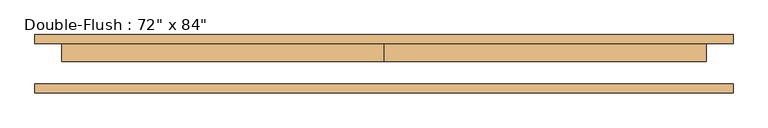
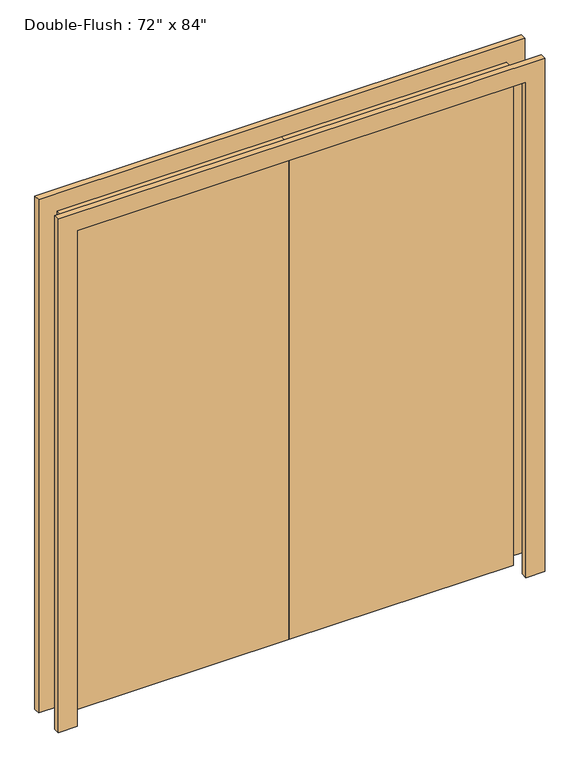
"""IFC4 building model written with IfcOpenShell, lengths in millimetres: door geometry."""

from ifc_helpers import new_model, si_unit, frame, origin, origin_with_axes, place, context, project, spatial, polyline, outline, extrude, source, transform, mapped, element, save


def door_3e29e47a(model_context):
    return source(origin(), model_context, "Body", "SweptSolid", [
        extrude(outline(polyline([(0.0, 57.15), (914.4, 57.15), (914.4, 6.35), (0.0, 6.35), (0.0, 57.15)])), origin_with_axes(), (0.0, 0.0, 1.0), 2133.6),
        extrude(outline(polyline([(-914.4, 57.15), (0.0, 57.15), (0.0, 6.35), (-914.4, 6.35), (-914.4, 57.15)])), origin_with_axes(), (0.0, 0.0, 1.0), 2133.6),
        extrude(outline(polyline([(2133.6, -914.4), (2133.6, 914.4), (0.0, 914.4), (0.0, 990.6), (2209.8, 990.6), (2209.8, -990.6), (0.0, -990.6), (0.0, -914.4), (2133.6, -914.4)])), frame((0.0, -82.55, 0.0), z_axis=(0.0, 1.0, 0.0), x_axis=(0.0, 0.0, 1.0)), (0.0, 0.0, 1.0), 25.4),
        extrude(outline(polyline([(2133.6, -914.4), (2133.6, 914.4), (0.0, 914.4), (0.0, 990.6), (2209.8, 990.6), (2209.8, -990.6), (0.0, -990.6), (0.0, -914.4), (2133.6, -914.4)])), frame((0.0, 57.15, 0.0), z_axis=(0.0, 1.0, 0.0), x_axis=(0.0, 0.0, 1.0)), (0.0, 0.0, 1.0), 25.4),
    ])


if __name__ == "__main__":
    model = new_model("IFC4")
    model_context = context("Model", 3, world=origin())
    ifc_project = project(units=[si_unit("LENGTHUNIT", "METRE", prefix="MILLI")], contexts=[model_context])
    site = spatial("IfcSite", under=ifc_project)
    building = spatial("IfcBuilding", under=site)
    placement = place(None, origin())
    door_shape = door_3e29e47a(model_context)
    element("IfcDoor", 1, ObjectType="Double-Flush : 72\" x 84\"", at=placement, inside=building, context=model_context, shape_type="MappedRepresentation", body=[
        mapped(door_shape, transform((0.0, 0.0, 0.0), x_axis=(1.0, 0.0, 0.0), y_axis=(0.0, 1.0, 0.0), z_axis=(0.0, 0.0, 1.0))),
    ])
    save(model, "model.ifc")

# Revit data of these elements
# Type "Double-Flush : 72\" x 84\""
#   Type Mark = "12"
#   Assembly Code = "C1020"
#   Thickness = 0' - 2"
#   Height = 7' - 0"
#   Trim Projection Ext = 0' - 1"
#   Trim Projection Int = 0' - 1"
#   Trim Width = 0' - 3"
#   Width = 6' - 0"
#   Function = 0
#   Door Material = Door - Panel
#   Frame Material = Door - Frame
#   Wall Closure = (empty or 0)
# Element 1 (IfcDoor, "Double-Flush : 72\" x 84\"")
#   Materials on its faces: "Door - Frame", "Door - Panel"
# Materials
#   "Door - Panel": class "Wood", colour RGB 210 159 95, transparency 0
#   "Door - Frame": class "Miscellaneous", colour RGB 118 70 51, transparency 0
